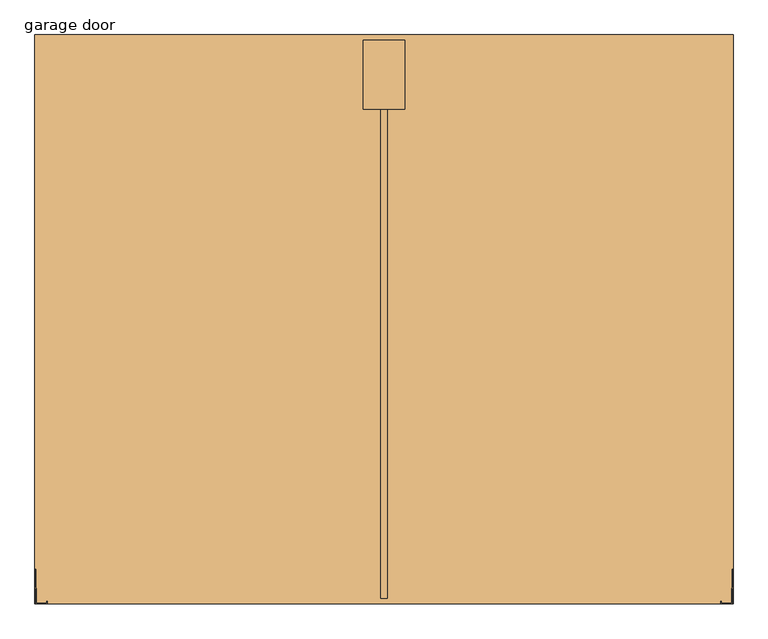
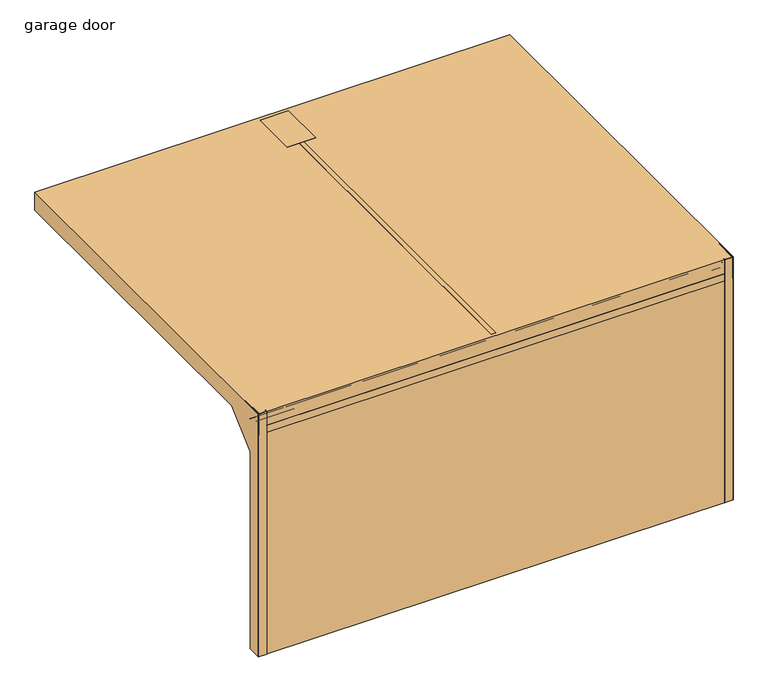
"""IFC4 building model written with IfcOpenShell, lengths in millimetres: door geometry, Sectional_Door_LPU_RU : garage door."""

from ifc_helpers import new_model, si_unit, point, frame, frame_2d, origin, origin_with_axes, place, context, project, spatial, polyline, circle_curve, trimmed, segment, composite_curve, outline, extrude, faceted_brep, source, transform, mapped, element, save
from ifc_brep_helpers import plane_surface, cylinder_surface, revolved_surface, advanced_brep


def garage_door_3c0e62b6(model_context):
    return source(origin(), model_context, "Body", "SolidModel", [
        extrude(outline(polyline([(-1601.2472293, 2039.6377448), (-1628.6278097, 2039.6377448), (-1628.6278097, 2002.03125), (-1637.0303432, 2002.03125), (-1637.0303432, 2490.0), (-1629.0303432, 2490.0), (-1629.0303432, 2512.7083202), (-1605.0303432, 2535.1762842), (-1605.0303432, 2490.0), (-1595.0303432, 2490.0), (-1595.0303432, 2015.0), (-1601.2472293, 2015.0), (-1601.2472293, 2039.6377448)])), frame((-2458.4, 0.0, 0.0), z_axis=(1.0, 0.0, 0.0), x_axis=(0.0, 1.0, 0.0)), (0.0, 0.0, 1.0), 4916.8),
        extrude(outline(polyline([(-1601.2472293, 1539.6377448), (-1628.6278097, 1539.6377448), (-1628.6278097, 1502.03125), (-1637.0303432, 1502.03125), (-1637.0303432, 1990.0), (-1629.0303432, 1990.0), (-1629.0303432, 2012.7083202), (-1605.0303432, 2035.1762842), (-1605.0303432, 1990.0), (-1595.0303432, 1990.0), (-1595.0303432, 1515.0), (-1601.2472293, 1515.0), (-1601.2472293, 1539.6377448)])), frame((-2458.4, 0.0, 0.0), z_axis=(1.0, 0.0, 0.0), x_axis=(0.0, 1.0, 0.0)), (0.0, 0.0, 1.0), 4916.8),
        extrude(outline(polyline([(-1601.2472293, 1039.6377448), (-1628.6278097, 1039.6377448), (-1628.6278097, 1002.03125), (-1637.0303432, 1002.03125), (-1637.0303432, 1490.0), (-1629.0303432, 1490.0), (-1629.0303432, 1512.7083202), (-1605.0303432, 1535.1762842), (-1605.0303432, 1490.0), (-1595.0303432, 1490.0), (-1595.0303432, 1015.0), (-1601.2472293, 1015.0), (-1601.2472293, 1039.6377448)])), frame((-2458.4, 0.0, 0.0), z_axis=(1.0, 0.0, 0.0), x_axis=(0.0, 1.0, 0.0)), (0.0, 0.0, 1.0), 4916.8),
        extrude(outline(polyline([(-1601.2472293, 539.6377448), (-1628.6278097, 539.6377448), (-1628.6278097, 502.03125), (-1637.0303432, 502.03125), (-1637.0303432, 990.0), (-1629.0303432, 990.0), (-1629.0303432, 1012.7083202), (-1605.0303432, 1035.1762842), (-1605.0303432, 990.0), (-1595.0303432, 990.0), (-1595.0303432, 515.0), (-1601.2472293, 515.0), (-1601.2472293, 539.6377448)])), frame((-2458.4, 0.0, 0.0), z_axis=(1.0, 0.0, 0.0), x_axis=(0.0, 1.0, 0.0)), (0.0, 0.0, 1.0), 4916.8),
        extrude(outline(polyline([(-150.0, 2425.9696568), (150.0, 2425.9696568), (150.0, 1925.9696568), (-150.0, 1925.9696568), (-150.0, 2425.9696568)])), frame((0.0, 0.0, 2595.0), z_axis=(0.0, 0.0, 1.0), x_axis=(1.0, 0.0, 0.0)), (0.0, 0.0, 1.0), 140.0),
        extrude(outline(polyline([(2523.4003172, -1659.0303432), (2438.4, -1659.0303432), (2438.4, -1638.7178432), (2441.7654545, -1638.7178432), (2441.7654545, -1655.2208416), (2519.9628172, -1655.2208416), (2519.9628172, -1544.4759666), (2524.739741, -1539.6990428), (2528.2752749, -1543.2345767), (2523.4003172, -1548.1095345), (2523.4003172, -1659.0303432)])), origin_with_axes(), (0.0, 0.0, 1.0), 2735.0),
        extrude(outline(polyline([(-2523.4003172, -1659.0303432), (-2523.4003172, -1548.1095345), (-2528.2752749, -1543.2345767), (-2524.739741, -1539.6990428), (-2519.9628172, -1544.4759666), (-2519.9628172, -1655.2208416), (-2441.7654545, -1655.2208416), (-2441.7654545, -1638.7178432), (-2438.4, -1638.7178432), (-2438.4, -1659.0303432), (-2523.4003172, -1659.0303432)])), origin_with_axes(), (0.0, 0.0, 1.0), 2735.0),
        extrude(outline(polyline([(-1408.7178432, 2735.0), (-1408.7178432, 2595.0), (-1548.1095345, 2494.9608265), (-1659.0303432, 2494.9608265), (-1659.0303432, 2735.0), (-1408.7178432, 2735.0)])), frame((2523.4003172, 0.0, 0.0), z_axis=(1.0, 0.0, 0.0), x_axis=(0.0, 1.0, 0.0)), (0.0, 0.0, 1.0), 3.7125221),
        extrude(outline(polyline([(-1408.7178432, 2735.0), (-1408.7178432, 2595.0), (-1548.1095345, 2494.9608265), (-1659.0303432, 2494.9608265), (-1659.0303432, 2735.0), (-1408.7178432, 2735.0)])), frame((-2527.1128393, 0.0, 0.0), z_axis=(1.0, 0.0, 0.0), x_axis=(0.0, 1.0, 0.0)), (0.0, 0.0, 1.0), 3.7125221),
        extrude(outline(polyline([(2518.4, 1286.6844584), (-2518.4, 1286.6844584), (-2518.4, 1351.6844584), (2518.4, 1351.6844584), (2518.4, 1286.6844584)])), frame((0.0, 0.0, 2687.5), z_axis=(0.0, 0.0, 1.0), x_axis=(1.0, 0.0, 0.0)), (0.0, 0.0, 1.0), 2.5),
        extrude(outline(polyline([(-1659.0303432, 2580.0), (-1638.737141, 2580.0), (-1638.737141, 2565.0), (-1640.5687539, 2565.0), (-1640.5687539, 2577.8988964), (-1657.1312539, 2577.8988964), (-1657.1312539, 2502.7049207), (-1640.5687539, 2502.7049207), (-1640.5687539, 2515.838061), (-1638.737141, 2515.838061), (-1638.737141, 2500.0), (-1659.0303432, 2500.0), (-1659.0303432, 2580.0)])), frame((-2438.4, 0.0, 0.0), z_axis=(1.0, 0.0, 0.0), x_axis=(0.0, 1.0, 0.0)), (0.0, 0.0, 1.0), 4876.8),
        faceted_brep([(-2488.4, -1636.7431471, 2607.219103), (-2518.4, -1636.7431471, 2607.219103), (-2518.4, -1601.2258031, 2552.780897), (-2488.4, -1601.2258031, 2552.780897), (-2488.4, -1607.025551, 2561.6702968), (-2490.8606703, -1607.025551, 2561.6702968), (-2490.8606703, -1602.9273959, 2555.3889654), (-2515.8606703, -1602.9273959, 2555.3889654), (-2515.8606703, -1635.7126366, 2605.6396171), (-2490.8606703, -1635.7126366, 2605.6396171), (-2490.8606703, -1631.2789403, 2598.8439944), (-2488.4, -1631.2789403, 2598.8439944), (-2488.4, 1350.9696568, 2687.5), (-2488.4, 1350.9696568, 2677.5), (-2490.8606703, 1350.9696568, 2677.5), (-2490.8606703, 1350.9696568, 2685.6140711), (-2515.8606703, 1350.9696568, 2685.6140711), (-2515.8606703, 1350.9696568, 2625.6140711), (-2490.8606703, 1350.9696568, 2625.6140711), (-2490.8606703, 1350.9696568, 2633.1140711), (-2488.4, 1350.9696568, 2633.1140711), (-2488.4, 1350.9696568, 2622.5), (-2518.4, 1350.9696568, 2622.5), (-2518.4, 1350.9696568, 2687.5), (-2490.8606703, -1510.7211691, 2677.5), (-2488.4, -1510.7211691, 2677.5), (-2515.8606703, -1513.1340507, 2685.6140711), (-2490.8606703, -1513.1340507, 2685.6140711), (-2490.8606703, -1495.2918483, 2625.6140711), (-2515.8606703, -1495.2918483, 2625.6140711), (-2488.4, -1497.5221236, 2633.1140711), (-2490.8606703, -1497.5221236, 2633.1140711), (-2518.4, -1494.3658169, 2622.5), (-2488.4, -1494.3658169, 2622.5), (-2488.4, -1513.6948695, 2687.5), (-2518.4, -1513.6948695, 2687.5)], [[[0, 1, 2, 3, 4, 5, 6, 7, 8, 9, 10, 11]], [[12, 13, 14, 15, 16, 17, 18, 19, 20, 21, 22, 23]], [[24, 14, 13, 25]], [[26, 16, 15, 27]], [[28, 18, 17, 29]], [[30, 20, 19, 31]], [[32, 22, 21, 33]], [[34, 12, 23, 35]], [[11, 25, 13, 12, 34, 0]], [[10, 24, 25, 11]], [[9, 27, 15, 14, 24, 10]], [[8, 26, 27, 9]], [[7, 29, 17, 16, 26, 8]], [[6, 28, 29, 7]], [[5, 31, 19, 18, 28, 6]], [[4, 30, 31, 5]], [[3, 33, 21, 20, 30, 4]], [[2, 32, 33, 3]], [[1, 35, 23, 22, 32, 2]], [[0, 34, 35, 1]]]),
        faceted_brep([(2488.4, -1636.7431471, 2607.219103), (2488.4, -1631.2789403, 2598.8439944), (2490.8606703, -1631.2789403, 2598.8439944), (2490.8606703, -1635.7126366, 2605.6396171), (2515.8606703, -1635.7126366, 2605.6396171), (2515.8606703, -1602.9273959, 2555.3889654), (2490.8606703, -1602.9273959, 2555.3889654), (2490.8606703, -1607.025551, 2561.6702968), (2488.4, -1607.025551, 2561.6702968), (2488.4, -1601.2258031, 2552.780897), (2518.4, -1601.2258031, 2552.780897), (2518.4, -1636.7431471, 2607.219103), (2488.4, 1350.9696568, 2687.5), (2518.4, 1350.9696568, 2687.5), (2518.4, 1350.9696568, 2622.5), (2488.4, 1350.9696568, 2622.5), (2488.4, 1350.9696568, 2633.1140711), (2490.8606703, 1350.9696568, 2633.1140711), (2490.8606703, 1350.9696568, 2625.6140711), (2515.8606703, 1350.9696568, 2625.6140711), (2515.8606703, 1350.9696568, 2685.6140711), (2490.8606703, 1350.9696568, 2685.6140711), (2490.8606703, 1350.9696568, 2677.5), (2488.4, 1350.9696568, 2677.5), (2518.4, -1513.6948695, 2687.5), (2488.4, -1513.6948695, 2687.5), (2488.4, -1494.3658169, 2622.5), (2518.4, -1494.3658169, 2622.5), (2490.8606703, -1497.5221236, 2633.1140711), (2488.4, -1497.5221236, 2633.1140711), (2515.8606703, -1495.2918483, 2625.6140711), (2490.8606703, -1495.2918483, 2625.6140711), (2490.8606703, -1513.1340507, 2685.6140711), (2515.8606703, -1513.1340507, 2685.6140711), (2488.4, -1510.7211691, 2677.5), (2490.8606703, -1510.7211691, 2677.5)], [[[0, 1, 2, 3, 4, 5, 6, 7, 8, 9, 10, 11]], [[12, 13, 14, 15, 16, 17, 18, 19, 20, 21, 22, 23]], [[24, 13, 12, 25]], [[26, 15, 14, 27]], [[28, 17, 16, 29]], [[30, 19, 18, 31]], [[32, 21, 20, 33]], [[34, 23, 22, 35]], [[11, 24, 25, 0]], [[10, 27, 14, 13, 24, 11]], [[9, 26, 27, 10]], [[8, 29, 16, 15, 26, 9]], [[7, 28, 29, 8]], [[6, 31, 18, 17, 28, 7]], [[5, 30, 31, 6]], [[4, 33, 20, 19, 30, 5]], [[3, 32, 33, 4]], [[2, 35, 22, 21, 32, 3]], [[1, 34, 35, 2]], [[0, 25, 12, 23, 34, 1]]]),
        advanced_brep(
        [(2488.4, -1616.5303432, 0.0), (2488.4, -1606.5303432, 0.0), (2490.8606703, -1606.5303432, 0.0), (2490.8606703, -1614.6444143, 0.0), (2515.8606703, -1614.6444143, 0.0), (2515.8606703, -1554.6444143, 0.0), (2490.8606703, -1554.6444143, 0.0), (2490.8606703, -1562.1444143, 0.0), (2488.4, -1562.1444143, 0.0), (2488.4, -1551.5303432, 0.0), (2518.4, -1551.5303432, 0.0), (2518.4, -1616.5303432, 0.0), (2488.4, -1562.1444143, 2280.0), (2488.4, -1284.0303432, 2558.1140711), (2488.4, 1350.9696568, 2558.1140711), (2488.4, 1350.9696568, 2547.5), (2488.4, -1284.0303432, 2547.5), (2488.4, -1551.5303432, 2280.0), (2490.8606703, -1562.1444143, 2280.0), (2490.8606703, -1284.0303432, 2558.1140711), (2488.4, 1350.9696568, 2612.5), (2518.4, 1350.9696568, 2612.5), (2518.4, 1350.9696568, 2547.5), (2490.8606703, 1350.9696568, 2558.1140711), (2490.8606703, 1350.9696568, 2550.6140711), (2515.8606703, 1350.9696568, 2550.6140711), (2515.8606703, 1350.9696568, 2610.6140711), (2490.8606703, 1350.9696568, 2610.6140711), (2490.8606703, 1350.9696568, 2602.5), (2488.4, 1350.9696568, 2602.5), (2488.4, -1616.5303432, 2280.0), (2488.4, -1284.0303432, 2612.5), (2488.4, -1284.0303432, 2602.5), (2488.4, -1606.5303432, 2280.0), (2490.8606703, -1606.5303432, 2280.0), (2490.8606703, -1284.0303432, 2602.5), (2490.8606703, -1284.0303432, 2610.6140711), (2490.8606703, -1614.6444143, 2280.0), (2515.8606703, -1614.6444143, 2280.0), (2515.8606703, -1284.0303432, 2610.6140711), (2515.8606703, -1284.0303432, 2550.6140711), (2515.8606703, -1554.6444143, 2280.0), (2490.8606703, -1554.6444143, 2280.0), (2490.8606703, -1284.0303432, 2550.6140711), (2518.4, -1551.5303432, 2280.0), (2518.4, -1284.0303432, 2547.5), (2518.4, -1284.0303432, 2612.5), (2518.4, -1616.5303432, 2280.0)],
        [
            (0, 1),
            (1, 2),
            (2, 3),
            (3, 4),
            (4, 5),
            (5, 6),
            (6, 7),
            (7, 8),
            (8, 9),
            (9, 10),
            (10, 11),
            (11, 0),
            (8, 12),
            (12, 13, circle_curve(frame((2488.4, -1284.0303432, 2280.0), z_axis=(-1.0, 0.0, 0.0), x_axis=(0.0, -1.0, 0.0)), 278.1140711)),
            (13, 14),
            (14, 15),
            (15, 16),
            (16, 17, circle_curve(frame((2488.4, -1284.0303432, 2280.0), z_axis=(1.0, 0.0, 0.0), x_axis=(0.0, -1.0, 0.0)), 267.5)),
            (17, 9),
            (7, 18),
            (18, 12),
            (19, 13),
            (18, 19, circle_curve(frame((2490.8606703, -1284.0303432, 2280.0), z_axis=(-1.0, 0.0, 0.0), x_axis=(0.0, -1.0, 0.0)), 278.1140711)),
            (20, 21),
            (21, 22),
            (22, 15),
            (14, 23),
            (23, 24),
            (24, 25),
            (25, 26),
            (26, 27),
            (27, 28),
            (28, 29),
            (29, 20),
            (19, 23),
            (0, 30),
            (30, 31, circle_curve(frame((2488.4, -1284.0303432, 2280.0), z_axis=(-1.0, 0.0, 0.0), x_axis=(0.0, -1.0, 0.0)), 332.5)),
            (31, 20),
            (29, 32),
            (32, 33, circle_curve(frame((2488.4, -1284.0303432, 2280.0), z_axis=(1.0, 0.0, 0.0), x_axis=(0.0, -1.0, 0.0)), 322.5)),
            (33, 1),
            (33, 34),
            (34, 2),
            (34, 35, circle_curve(frame((2490.8606703, -1284.0303432, 2280.0), z_axis=(-1.0, 0.0, 0.0), x_axis=(0.0, -1.0, 0.0)), 322.5)),
            (35, 28),
            (27, 36),
            (36, 37, circle_curve(frame((2490.8606703, -1284.0303432, 2280.0), z_axis=(1.0, 0.0, 0.0), x_axis=(0.0, -1.0, 0.0)), 330.6140711)),
            (37, 3),
            (37, 38),
            (38, 4),
            (38, 39, circle_curve(frame((2515.8606703, -1284.0303432, 2280.0), z_axis=(-1.0, 0.0, 0.0), x_axis=(0.0, -1.0, 0.0)), 330.6140711)),
            (39, 26),
            (25, 40),
            (40, 41, circle_curve(frame((2515.8606703, -1284.0303432, 2280.0), z_axis=(1.0, 0.0, 0.0), x_axis=(0.0, -1.0, 0.0)), 270.6140711)),
            (41, 5),
            (41, 42),
            (42, 6),
            (42, 43, circle_curve(frame((2490.8606703, -1284.0303432, 2280.0), z_axis=(-1.0, 0.0, 0.0), x_axis=(0.0, -1.0, 0.0)), 270.6140711)),
            (43, 24),
            (17, 44),
            (44, 10),
            (44, 45, circle_curve(frame((2518.4, -1284.0303432, 2280.0), z_axis=(-1.0, 0.0, 0.0), x_axis=(0.0, -1.0, 0.0)), 267.5)),
            (45, 22),
            (21, 46),
            (46, 47, circle_curve(frame((2518.4, -1284.0303432, 2280.0), z_axis=(1.0, 0.0, 0.0), x_axis=(0.0, -1.0, 0.0)), 332.5)),
            (47, 11),
            (47, 30),
            (32, 35),
            (36, 39),
            (40, 43),
            (16, 45),
            (46, 31),
        ],
        [
            plane_surface(frame((2438.4, -1584.0303432, 0.0), z_axis=(0.0, 0.0, -1.0), x_axis=(1.0, 0.0, 0.0))),
            plane_surface(frame((2488.4, -1551.5303432, 0.0), z_axis=(-1.0, 0.0, 0.0), x_axis=(0.0, 0.0, 1.0))),
            plane_surface(frame((2488.4, -1562.1444143, 0.0), z_axis=(0.0, -1.0, 0.0), x_axis=(0.0, 0.0, 1.0))),
            cylinder_surface(frame((2438.4, -1284.0303432, 2280.0), z_axis=(1.0, 0.0, 0.0), x_axis=(0.0, -1.0, 0.0)), 278.1140711),
            plane_surface(frame((2438.4, 1350.9696568, 2580.0), z_axis=(0.0, 1.0, 0.0), x_axis=(1.0, 0.0, 0.0))),
            plane_surface(frame((2488.4, -1284.0303432, 2558.1140711), z_axis=(0.0, 0.0, 1.0), x_axis=(0.0, 1.0, 0.0))),
            plane_surface(frame((2488.4, -1606.5303432, 0.0), z_axis=(-1.0, 0.0, 0.0), x_axis=(0.0, 0.0, 1.0))),
            plane_surface(frame((2490.8606703, -1606.5303432, 0.0), z_axis=(0.0, 1.0, 0.0), x_axis=(0.0, 0.0, 1.0))),
            plane_surface(frame((2490.8606703, -1614.6444143, 0.0), z_axis=(1.0, 0.0, 0.0), x_axis=(0.0, 0.0, 1.0))),
            plane_surface(frame((2515.8606703, -1614.6444143, 0.0), z_axis=(0.0, 1.0, 0.0), x_axis=(0.0, 0.0, 1.0))),
            plane_surface(frame((2515.8606703, -1554.6444143, 0.0), z_axis=(-1.0, 0.0, 0.0), x_axis=(0.0, 0.0, 1.0))),
            plane_surface(frame((2490.8606703, -1554.6444143, 0.0), z_axis=(0.0, -1.0, 0.0), x_axis=(0.0, 0.0, 1.0))),
            plane_surface(frame((2490.8606703, -1562.1444143, 0.0), z_axis=(1.0, 0.0, 0.0), x_axis=(0.0, 0.0, 1.0))),
            plane_surface(frame((2518.4, -1551.5303432, 0.0), z_axis=(0.0, 1.0, 0.0), x_axis=(0.0, 0.0, 1.0))),
            plane_surface(frame((2518.4, -1616.5303432, 0.0), z_axis=(1.0, 0.0, 0.0), x_axis=(0.0, 0.0, 1.0))),
            plane_surface(frame((2488.4, -1616.5303432, 0.0), z_axis=(0.0, -1.0, 0.0), x_axis=(0.0, 0.0, 1.0))),
            revolved_surface(polyline([(2490.8606703, -1606.5303432, 2280.0), (2488.4, -1606.5303432, 2280.0)]), (2438.4, -1284.0303432, 2280.0), (1.0, 0.0, 0.0)),
            revolved_surface(polyline([(2515.8606703, -1614.6444143, 2280.0), (2490.8606703, -1614.6444143, 2280.0)]), (2438.4, -1284.0303432, 2280.0), (1.0, 0.0, 0.0)),
            cylinder_surface(frame((2438.4, -1284.0303432, 2280.0), z_axis=(1.0, 0.0, 0.0), x_axis=(0.0, -1.0, 0.0)), 270.6140711),
            revolved_surface(polyline([(2518.4, -1551.5303432, 2280.0), (2488.4, -1551.5303432, 2280.0)]), (2438.4, -1284.0303432, 2280.0), (1.0, 0.0, 0.0)),
            cylinder_surface(frame((2438.4, -1284.0303432, 2280.0), z_axis=(1.0, 0.0, 0.0), x_axis=(0.0, -1.0, 0.0)), 332.5),
            plane_surface(frame((2490.8606703, -1284.0303432, 2602.5), z_axis=(0.0, 0.0, -1.0), x_axis=(0.0, 1.0, 0.0))),
            plane_surface(frame((2515.8606703, -1284.0303432, 2610.6140711), z_axis=(0.0, 0.0, -1.0), x_axis=(0.0, 1.0, 0.0))),
            plane_surface(frame((2490.8606703, -1284.0303432, 2550.6140711), z_axis=(0.0, 0.0, 1.0), x_axis=(0.0, 1.0, 0.0))),
            plane_surface(frame((2518.4, -1284.0303432, 2547.5), z_axis=(0.0, 0.0, -1.0), x_axis=(0.0, 1.0, 0.0))),
            plane_surface(frame((2488.4, -1284.0303432, 2612.5), z_axis=(0.0, 0.0, 1.0), x_axis=(0.0, 1.0, 0.0))),
        ],
        [
            (0, [[1, 2, 3, 4, 5, 6, 7, 8, 9, 10, 11, 12]]),
            (1, [[13, 14, 15, 16, 17, 18, 19, -9]]),
            (2, [[20, 21, -13, -8]]),
            (3, [[22, -14, -21, 23]]),
            (4, [[24, 25, 26, -16, 27, 28, 29, 30, 31, 32, 33, 34]]),
            (5, [[35, -27, -15, -22]]),
            (6, [[36, 37, 38, -34, 39, 40, 41, -1]]),
            (7, [[-41, 42, 43, -2]]),
            (8, [[-43, 44, 45, -32, 46, 47, 48, -3]]),
            (9, [[-48, 49, 50, -4]]),
            (10, [[-50, 51, 52, -30, 53, 54, 55, -5]]),
            (11, [[-55, 56, 57, -6]]),
            (12, [[-57, 58, 59, -28, -35, -23, -20, -7]]),
            (13, [[-19, 60, 61, -10]]),
            (14, [[-61, 62, 63, -25, 64, 65, 66, -11]]),
            (15, [[-66, 67, -36, -12]]),
            (16, [[68, -44, -42, -40]]),
            (17, [[69, -51, -49, -47]]),
            (18, [[70, -58, -56, -54]]),
            (19, [[71, -62, -60, -18]]),
            (20, [[72, -37, -67, -65]]),
            (21, [[-39, -33, -45, -68]]),
            (22, [[-46, -31, -52, -69]]),
            (23, [[-53, -29, -59, -70]]),
            (24, [[-17, -26, -63, -71]]),
            (25, [[-64, -24, -38, -72]]),
        ],
    ),
        advanced_brep(
        [(-2488.4, -1616.5303432, 0.0), (-2518.4, -1616.5303432, 0.0), (-2518.4, -1551.5303432, 0.0), (-2488.4, -1551.5303432, 0.0), (-2488.4, -1562.1444143, 0.0), (-2490.8606703, -1562.1444143, 0.0), (-2490.8606703, -1554.6444143, 0.0), (-2515.8606703, -1554.6444143, 0.0), (-2515.8606703, -1614.6444143, 0.0), (-2490.8606703, -1614.6444143, 0.0), (-2490.8606703, -1606.5303432, 0.0), (-2488.4, -1606.5303432, 0.0), (-2518.4, -1616.5303432, 2280.0), (-2518.4, -1284.0303432, 2612.5), (-2518.4, 1350.9696568, 2612.5), (-2518.4, 1350.9696568, 2547.5), (-2518.4, -1284.0303432, 2547.5), (-2518.4, -1551.5303432, 2280.0), (-2488.4, -1551.5303432, 2280.0), (-2488.4, -1606.5303432, 2280.0), (-2488.4, -1284.0303432, 2602.5), (-2488.4, 1350.9696568, 2602.5), (-2488.4, 1350.9696568, 2612.5), (-2488.4, -1284.0303432, 2612.5), (-2488.4, -1616.5303432, 2280.0), (-2490.8606703, -1606.5303432, 2280.0), (-2490.8606703, -1614.6444143, 2280.0), (-2490.8606703, -1284.0303432, 2610.6140711), (-2490.8606703, 1350.9696568, 2610.6140711), (-2490.8606703, 1350.9696568, 2602.5), (-2490.8606703, -1284.0303432, 2602.5), (-2515.8606703, -1614.6444143, 2280.0), (-2515.8606703, -1554.6444143, 2280.0), (-2515.8606703, -1284.0303432, 2550.6140711), (-2515.8606703, 1350.9696568, 2550.6140711), (-2515.8606703, 1350.9696568, 2610.6140711), (-2515.8606703, -1284.0303432, 2610.6140711), (-2490.8606703, -1554.6444143, 2280.0), (-2490.8606703, -1562.1444143, 2280.0), (-2490.8606703, -1284.0303432, 2558.1140711), (-2490.8606703, 1350.9696568, 2558.1140711), (-2490.8606703, 1350.9696568, 2550.6140711), (-2490.8606703, -1284.0303432, 2550.6140711), (-2488.4, 1350.9696568, 2558.1140711), (-2488.4, 1350.9696568, 2547.5), (-2488.4, -1284.0303432, 2547.5), (-2488.4, -1562.1444143, 2280.0), (-2488.4, -1284.0303432, 2558.1140711)],
        [
            (0, 1),
            (1, 2),
            (2, 3),
            (3, 4),
            (4, 5),
            (5, 6),
            (6, 7),
            (7, 8),
            (8, 9),
            (9, 10),
            (10, 11),
            (11, 0),
            (1, 12),
            (12, 13, circle_curve(frame((-2518.4, -1284.0303432, 2280.0), z_axis=(-1.0, 0.0, 0.0), x_axis=(0.0, -1.0, 0.0)), 332.5)),
            (13, 14),
            (14, 15),
            (15, 16),
            (16, 17, circle_curve(frame((-2518.4, -1284.0303432, 2280.0), z_axis=(1.0, 0.0, 0.0), x_axis=(0.0, -1.0, 0.0)), 267.5)),
            (17, 2),
            (17, 18),
            (18, 3),
            (11, 19),
            (19, 20, circle_curve(frame((-2488.4, -1284.0303432, 2280.0), z_axis=(-1.0, 0.0, 0.0), x_axis=(0.0, -1.0, 0.0)), 322.5)),
            (20, 21),
            (21, 22),
            (22, 23),
            (23, 24, circle_curve(frame((-2488.4, -1284.0303432, 2280.0), z_axis=(1.0, 0.0, 0.0), x_axis=(0.0, -1.0, 0.0)), 332.5)),
            (24, 0),
            (10, 25),
            (25, 19),
            (9, 26),
            (26, 27, circle_curve(frame((-2490.8606703, -1284.0303432, 2280.0), z_axis=(-1.0, 0.0, 0.0), x_axis=(0.0, -1.0, 0.0)), 330.6140711)),
            (27, 28),
            (28, 29),
            (29, 30),
            (30, 25, circle_curve(frame((-2490.8606703, -1284.0303432, 2280.0), z_axis=(1.0, 0.0, 0.0), x_axis=(0.0, -1.0, 0.0)), 322.5)),
            (8, 31),
            (31, 26),
            (7, 32),
            (32, 33, circle_curve(frame((-2515.8606703, -1284.0303432, 2280.0), z_axis=(-1.0, 0.0, 0.0), x_axis=(0.0, -1.0, 0.0)), 270.6140711)),
            (33, 34),
            (34, 35),
            (35, 36),
            (36, 31, circle_curve(frame((-2515.8606703, -1284.0303432, 2280.0), z_axis=(1.0, 0.0, 0.0), x_axis=(0.0, -1.0, 0.0)), 330.6140711)),
            (6, 37),
            (37, 32),
            (5, 38),
            (38, 39, circle_curve(frame((-2490.8606703, -1284.0303432, 2280.0), z_axis=(-1.0, 0.0, 0.0), x_axis=(0.0, -1.0, 0.0)), 278.1140711)),
            (39, 40),
            (40, 41),
            (41, 42),
            (42, 37, circle_curve(frame((-2490.8606703, -1284.0303432, 2280.0), z_axis=(1.0, 0.0, 0.0), x_axis=(0.0, -1.0, 0.0)), 270.6140711)),
            (24, 12),
            (21, 29),
            (28, 35),
            (34, 41),
            (40, 43),
            (43, 44),
            (44, 15),
            (14, 22),
            (44, 45),
            (45, 16),
            (20, 30),
            (27, 36),
            (33, 42),
            (13, 23),
            (45, 18, circle_curve(frame((-2488.4, -1284.0303432, 2280.0), z_axis=(1.0, 0.0, 0.0), x_axis=(0.0, -1.0, 0.0)), 267.5)),
            (4, 46),
            (46, 38),
            (43, 47),
            (47, 46, circle_curve(frame((-2488.4, -1284.0303432, 2280.0), z_axis=(1.0, 0.0, 0.0), x_axis=(0.0, -1.0, 0.0)), 278.1140711)),
            (47, 39),
        ],
        [
            plane_surface(frame((-2438.4, -1584.0303432, 0.0), z_axis=(0.0, 0.0, -1.0), x_axis=(1.0, 0.0, 0.0))),
            plane_surface(frame((-2518.4, -1551.5303432, 0.0), z_axis=(-1.0, 0.0, 0.0), x_axis=(0.0, 0.0, 1.0))),
            plane_surface(frame((-2488.4, -1551.5303432, 0.0), z_axis=(0.0, 1.0, 0.0), x_axis=(0.0, 0.0, 1.0))),
            plane_surface(frame((-2488.4, -1616.5303432, 0.0), z_axis=(1.0, 0.0, 0.0), x_axis=(0.0, 0.0, 1.0))),
            plane_surface(frame((-2488.4, -1606.5303432, 0.0), z_axis=(0.0, 1.0, 0.0), x_axis=(0.0, 0.0, 1.0))),
            plane_surface(frame((-2490.8606703, -1606.5303432, 0.0), z_axis=(-1.0, 0.0, 0.0), x_axis=(0.0, 0.0, 1.0))),
            plane_surface(frame((-2490.8606703, -1614.6444143, 0.0), z_axis=(0.0, 1.0, 0.0), x_axis=(0.0, 0.0, 1.0))),
            plane_surface(frame((-2515.8606703, -1614.6444143, 0.0), z_axis=(1.0, 0.0, 0.0), x_axis=(0.0, 0.0, 1.0))),
            plane_surface(frame((-2515.8606703, -1554.6444143, 0.0), z_axis=(0.0, -1.0, 0.0), x_axis=(0.0, 0.0, 1.0))),
            plane_surface(frame((-2490.8606703, -1554.6444143, 0.0), z_axis=(-1.0, 0.0, 0.0), x_axis=(0.0, 0.0, 1.0))),
            plane_surface(frame((-2518.4, -1616.5303432, 0.0), z_axis=(0.0, -1.0, 0.0), x_axis=(0.0, 0.0, 1.0))),
            plane_surface(frame((-2438.4, 1350.9696568, 2580.0), z_axis=(0.0, 1.0, 0.0), x_axis=(1.0, 0.0, 0.0))),
            plane_surface(frame((-2488.4, -1284.0303432, 2547.5), z_axis=(0.0, 0.0, -1.0), x_axis=(0.0, 1.0, 0.0))),
            plane_surface(frame((-2488.4, -1284.0303432, 2602.5), z_axis=(0.0, 0.0, -1.0), x_axis=(0.0, 1.0, 0.0))),
            plane_surface(frame((-2490.8606703, -1284.0303432, 2610.6140711), z_axis=(0.0, 0.0, -1.0), x_axis=(0.0, 1.0, 0.0))),
            plane_surface(frame((-2515.8606703, -1284.0303432, 2550.6140711), z_axis=(0.0, 0.0, 1.0), x_axis=(0.0, 1.0, 0.0))),
            plane_surface(frame((-2518.4, -1284.0303432, 2612.5), z_axis=(0.0, 0.0, 1.0), x_axis=(0.0, 1.0, 0.0))),
            revolved_surface(polyline([(-2488.4, -1551.5303432, 2280.0), (-2518.4, -1551.5303432, 2280.0)]), (-2438.4, -1284.0303432, 2280.0), (1.0, 0.0, 0.0)),
            revolved_surface(polyline([(-2488.4, -1606.5303432, 2280.0), (-2490.8606703, -1606.5303432, 2280.0)]), (-2438.4, -1284.0303432, 2280.0), (1.0, 0.0, 0.0)),
            revolved_surface(polyline([(-2490.8606703, -1614.6444143, 2280.0), (-2515.8606703, -1614.6444143, 2280.0)]), (-2438.4, -1284.0303432, 2280.0), (1.0, 0.0, 0.0)),
            cylinder_surface(frame((-2438.4, -1284.0303432, 2280.0), z_axis=(1.0, 0.0, 0.0), x_axis=(0.0, -1.0, 0.0)), 270.6140711),
            cylinder_surface(frame((-2438.4, -1284.0303432, 2280.0), z_axis=(1.0, 0.0, 0.0), x_axis=(0.0, -1.0, 0.0)), 332.5),
            plane_surface(frame((-2490.8606703, -1562.1444143, 0.0), z_axis=(0.0, -1.0, 0.0), x_axis=(0.0, 0.0, 1.0))),
            plane_surface(frame((-2488.4, -1562.1444143, 0.0), z_axis=(1.0, 0.0, 0.0), x_axis=(0.0, 0.0, 1.0))),
            cylinder_surface(frame((-2438.4, -1284.0303432, 2280.0), z_axis=(1.0, 0.0, 0.0), x_axis=(0.0, -1.0, 0.0)), 278.1140711),
            plane_surface(frame((-2490.8606703, -1284.0303432, 2558.1140711), z_axis=(0.0, 0.0, 1.0), x_axis=(0.0, 1.0, 0.0))),
        ],
        [
            (0, [[1, 2, 3, 4, 5, 6, 7, 8, 9, 10, 11, 12]]),
            (1, [[13, 14, 15, 16, 17, 18, 19, -2]]),
            (2, [[-19, 20, 21, -3]]),
            (3, [[22, 23, 24, 25, 26, 27, 28, -12]]),
            (4, [[29, 30, -22, -11]]),
            (5, [[31, 32, 33, 34, 35, 36, -29, -10]]),
            (6, [[37, 38, -31, -9]]),
            (7, [[39, 40, 41, 42, 43, 44, -37, -8]]),
            (8, [[45, 46, -39, -7]]),
            (9, [[47, 48, 49, 50, 51, 52, -45, -6]]),
            (10, [[-28, 53, -13, -1]]),
            (11, [[-25, 54, -34, 55, -42, 56, -50, 57, 58, 59, -16, 60]]),
            (12, [[-17, -59, 61, 62]]),
            (13, [[-35, -54, -24, 63]]),
            (14, [[-43, -55, -33, 64]]),
            (15, [[-51, -56, -41, 65]]),
            (16, [[-26, -60, -15, 66]]),
            (17, [[-62, 67, -20, -18]]),
            (18, [[-63, -23, -30, -36]]),
            (19, [[-64, -32, -38, -44]]),
            (20, [[-65, -40, -46, -52]]),
            (21, [[-66, -14, -53, -27]]),
            (22, [[68, 69, -47, -5]]),
            (23, [[-21, -67, -61, -58, 70, 71, -68, -4]]),
            (24, [[72, -48, -69, -71]]),
            (25, [[-70, -57, -49, -72]]),
        ],
    ),
        extrude(outline(polyline([(25.0, -1618.9844751), (-25.0, -1618.9844751), (-25.0, 1925.9696568), (25.0, 1925.9696568), (25.0, -1618.9844751)])), frame((0.0, 0.0, 2705.0), z_axis=(0.0, 0.0, 1.0), x_axis=(1.0, 0.0, 0.0)), (0.0, 0.0, 1.0), 30.0),
        extrude(outline(composite_curve([segment(trimmed(circle_curve(frame_2d((-1479.0303432, 2580.0)), 10.0), [point((-1469.0303432, 2580.0))], [point((-1489.0303432, 2580.0))], False, "CARTESIAN"), True, "CONTINUOUS"), segment(trimmed(circle_curve(frame_2d((-1479.0303432, 2580.0)), 10.0), [point((-1489.0303432, 2580.0))], [point((-1469.0303432, 2580.0))], False, "CARTESIAN"), True, "CONTINUOUS")], self_intersect=False)), frame((-2518.4, 0.0, 0.0), z_axis=(1.0, 0.0, 0.0), x_axis=(0.0, 1.0, 0.0)), (0.0, 0.0, 1.0), 5036.8),
        extrude(outline(composite_curve([segment(trimmed(circle_curve(frame_2d((-1479.0303432, 2580.0)), 50.0), [point((-1429.0303432, 2580.0))], [point((-1529.0303432, 2580.0))], False, "CARTESIAN"), True, "CONTINUOUS"), segment(trimmed(circle_curve(frame_2d((-1479.0303432, 2580.0)), 50.0), [point((-1529.0303432, 2580.0))], [point((-1429.0303432, 2580.0))], False, "CARTESIAN"), True, "CONTINUOUS")], self_intersect=False)), frame((-2468.4, 0.0, 0.0), z_axis=(1.0, 0.0, 0.0), x_axis=(0.0, 1.0, 0.0)), (0.0, 0.0, 1.0), 400.0),
        extrude(outline(composite_curve([segment(trimmed(circle_curve(frame_2d((-1479.0303432, 2580.0)), 50.0), [point((-1429.0303432, 2580.0))], [point((-1529.0303432, 2580.0))], False, "CARTESIAN"), True, "CONTINUOUS"), segment(trimmed(circle_curve(frame_2d((-1479.0303432, 2580.0)), 50.0), [point((-1529.0303432, 2580.0))], [point((-1429.0303432, 2580.0))], False, "CARTESIAN"), True, "CONTINUOUS")], self_intersect=False)), frame((2068.4, 0.0, 0.0), z_axis=(1.0, 0.0, 0.0), x_axis=(0.0, 1.0, 0.0)), (0.0, 0.0, 1.0), 400.0),
        extrude(outline(polyline([(-1659.0303432, 2735.0), (2465.9696568, 2735.0), (2465.9696568, 2530.0), (-1169.0303432, 2530.0), (-1504.0303432, 2215.0), (-1504.0303432, 0.0), (-1659.0303432, 0.0), (-1659.0303432, 2735.0)])), frame((-2528.4, 0.0, 0.0), z_axis=(1.0, 0.0, 0.0), x_axis=(0.0, 1.0, 0.0)), (0.0, 0.0, 1.0), 5056.8),
        extrude(outline(polyline([(-1601.2472293, 39.6377448), (-1628.6278097, 39.6377448), (-1628.6278097, 2.03125), (-1637.0303432, 2.03125), (-1637.0303432, 490.0), (-1629.0303432, 490.0), (-1629.0303432, 512.7083202), (-1605.0303432, 535.1762842), (-1605.0303432, 490.0), (-1595.0303432, 490.0), (-1595.0303432, 15.0), (-1601.2472293, 15.0), (-1601.2472293, 39.6377448)])), frame((-2458.4, 0.0, 0.0), z_axis=(1.0, 0.0, 0.0), x_axis=(0.0, 1.0, 0.0)), (0.0, 0.0, 1.0), 4916.8),
    ])


if __name__ == "__main__":
    model = new_model("IFC4")
    model_context = context("Model", 3, world=origin())
    ifc_project = project(units=[si_unit("LENGTHUNIT", "METRE", prefix="MILLI")], contexts=[model_context])
    site = spatial("IfcSite", under=ifc_project)
    building = spatial("IfcBuilding", under=site)
    placement = place(None, origin())
    garage_door_shape = garage_door_3c0e62b6(model_context)
    element("IfcDoor", 1, ObjectType="Sectional_Door_LPU_RU : garage door", at=placement, inside=building, context=model_context, shape_type="MappedRepresentation", body=[
        mapped(garage_door_shape, transform((0.0, 0.0, 0.0), x_axis=(1.0, 0.0, 0.0), y_axis=(0.0, 1.0, 0.0), z_axis=(0.0, 0.0, 1.0))),
    ])
    save(model, "model.ifc")

# Revit data of these elements
# Type "Sectional_Door_LPU_RU : garage door"
#   Type Mark = "30"
#   hoermann_family_version = "202111"
#   bimsys_family_version = "202111261846"
#   Wärmeschutz = "1.4 W/(m²·K)"
#   Windlastklasse nach EN 12424 = "Класс 3 – (0,7 кН/м2 или 120 км/ч)"
#   Verglasung Typ = "Без остекления"
#   URL 3 = "https://www.hoermann.de/mediacenter/"
#   URL 2 = "https://architektenprogramm.hoermann.de/HAP/entry.php"
#   URL = "https://www.hoermann.de/"
#   Steuerung Typ = "с помощью ручных передатчиков"
#   Schlupftür Typ = "Без порога"
#   Schlupftür Schloss Typ = "Стандартный замок"
#   Schlupftür Panikfunktion Typ = "Отсутствует"
#   Schlupftür Obentürschließer Typ = "Производно – доводчик с шиной скольжения"
#   Schlupftür DIN Richtung Typ = "DIN правый"
#   Schlupftür Bänder Typ = "Скрытые петли"
#   Schlupftür Beschlag innen Typ = "Производно (нажимная ручка U-образной формы)"
#   Schlupftür Beschlag außen Typ = "Без нажимной ручки"
#   Schlupftür Beschlag Material Typ = "Пластмасса черного цвета"
#   Schlupftür Aufschlagsrichtung = "глядя наружу"
#   Schallschutz = "Отсутствует"
#   STLB Leistungsbereich = "Двери / Ворота - Металл"
#   STLB Gewerk = "31"
#   Model = "LPU 42, Секция «Гараж»"
#   Lamellen Tor innen Typ = "С оттиском Stucco"
#   Lamellen Tor außen Typ = "Вудгрейн"
#   Lamellen Profil Typ = "L-гофр"
#   Gewichtsausgleich = "Технология натяжения пружины"
#   Fire Rating = "Отсутствует"
#   Einbruchschutz = "Отсутствует"
#   Einbauort = "Наружные стены"
#   DIN 276 Kostengruppe = "334"
#   CAL_Antrieb = "SupraMatic"
#   Manufacturer = "HÖRMANN"
#   Beschlag Tor Typ = "N-направляющая"
#   Beschichtung Lamellen innen Typ = "RAL 9002"
#   Beschichtung Lamellen außen Typ = "RAL 9016"
#   Antrieb Typ = "Отсутствует"
#   Analytic Construction = "<Keine Auswahl>"
#   Versatz Beschlag Schlupftür = 0' - 3.14961"
#   Torblatt Stärke (Bautiefe) = 0' - 1.65354"
#   Sturzhöhe [instance default] = 0' - 8.26772"
#   Schlupftür Stärke (Bautiefe) = 0' - 1.65354"
#   Schlupftür Lichte Durchgangshöhe [instance default] = 6' - 4.9685"
#   Schlupftür Lichte Durchgangsbreite = 2' - 8.67717"
#   Schlupftür Höhe [instance default] = 6' - 4.9685"
#   Schlupftür Breite = 3' - 1.00787"
#   Schlupftür Bedienelement Höhe = 3' - 5.33858"
#   Platzbedarf Lagerseite = 0' - 0"
#   Platzbedarf Antriebsseite = 0' - 0"
#   Fußbodenaufbau = 0' - 0"
#   Deckenhöhe min. [instance default] = 8' - 10.69291"
#   CAL_MinHöhe = 6' - 1.8189"
#   CAL_MinBreite = 6' - 6.74016"
#   Blende oben Ansichtshöhe = 0' - 0"
#   Rough Height = 8' - 2.4252"
#   Rough Width = 16' - 0"
#   CAL_RasterBreite [instance default] = 1' - 10.8189"
#   CAL_Beschlagsart extra länge = 1' - 8.07874"
#   CAL_Beschlag Extra Abstand = 2' - 5.52756"
#   CAL_PanelPosTop [instance default] = 4' - 11.05512"
#   CAL_Schlupftüre Position - Real [instance default] = 6' - 8.69291"
#   CAL_Schlupftüre Position - Kalkuliert [instance default] = 6' - 8.69291"
#   CAL_Beschlag Schlupftüre Position [instance default] = 2' - 8.71654"
#   CAL_Versatz Schlupftüre [instance default] = 4' - 6.67717"
#   CAL_PanelH_Min = 1' - 1.77953"
#   CAL_PanelH_Max = 3' - 7.30709"
#   CAL_Lamellen seitliche Überlappung = 0' - 0.7874"
#   CAL_Panel Tiefe = 0' - 1.65354"
#   CAL_Panel max. Breite [instance default] = 2' - 6.69291"
#   CAL_Panel Breite [instance default] = 16' - 1.5748"
#   CAL_Lamellen Höhe [instance default] = 1' - 7.68504"
#   CAL_Paneel Wandabstand = 0' - 0.86614"
#   CAL_Antrieb Abstand von Öffnungkopf [instance default] = 0' - 8.46457"
#   CAL_Antrieb Beschlag Breite = 0' - 1.1811"
#   CAL_Antrieb Beschlag Tiefe = 0' - 2.75591"
#   CAL_MaxGrößeSchlupftüre = 13' - 1.48031"
#   CAL_MaxBreite = 19' - 8.22047"
#   CAL_MaxHöhe = 9' - 10.11024"
#   CAL_GlasPanVerPos [instance default] = 3' - 3.37008"
#   Height = 8' - 2.4252"
#   CAL_Extra Horizontal Abstand = 3' - 3.37008"
#   Width = 16' - 0"
#   Verglasung ab Lamelle = 3
#   Verglasung Anzahl verglaster Lamellen = 1
#   Torglieder Anzahl = 5
#   ThermoFrame = no
#   Schlupftüranordnung = 2
#   Замок калитки, тип Id = 1
#   Калитка, функция «антипаника», тип Id = 1
#   Калитка, верхний доводчик, тип Id = 1
#   Калитка, направление открывания по DIN, тип Id = 1
#   Калитка, фурнитура, материал, тип Id = 1
#   Schlupftür = no
#   Minimalen Platzbedarf anzeigen [instance default] = yes
#   CE-Kennzeichen vorhanden = yes
#   Направляющая, ворота, тип Id = 3
#   CAL_TopPanelArray [instance default] = no
#   CAL_Größenwarnung [instance default] = no
#   CAL_FensterPanelAn [instance default] = no
#   CAL_OberPanelSingleAn [instance default] = no
#   CAL_OberPanelReiheAn [instance default] = no
#   CAL_Fehlermeldung anzeigen [instance default] = yes
#   Калитка, фурнитура внутри, тип Id = 1
#   CAL_Schlupftüre für Größe = yes
#   CAL_Fehler Schlupftüre [instance default] = no
#   CAL_Schlupftüre  - Real = no
#   CAL_PanelRasterNumTypeS [instance default] = 8
#   CAL_PanelRasterNumTypeM [instance default] = 6
#   CAL_PanelRasterNumTypeL [instance default] = 4
#   CAL_PanelRasterNumTypeD [instance default] = 5
#   CAL_PanelRasterNum [instance default] = 8
#   CAL_PanelNumberTop - Real [instance default] = 2
#   CAL_PanelNumberBottom - Real [instance default] = 5
#   CAL_Schlupftüre Links [instance default] = no
#   CAL_PanelNumber - Real [instance default] = 5
#   Секции, профиль, тип Id = 1
#   Калитка, фурнитура снаружи, тип Id = 1
#   CAL_Antrieb Id = 1
#   Остекление, тип Id = 0
#   CAL_Fehlermeldung sichtbar [instance default] = no
#   CAL_Schlupftüre für Typ = yes
#   CAL_UnterPanelEinzel = no
#   CAL_UnterPanelReihe = yes
#   Покрытие секций изнутри, тип Id = 1
#   Покрытие секций снаружи, тип Id = 1
#   Тип привода Id = 1
#   Zarge Material = Hörmann - RAL 9002
#   Schlupftür Beschlag Oberfläche = Hörmann - RAL 7004
#   Lamellen Material = Wall Texture, Stucco
#   CAL_Glaspanel Typ LPU [instance default] = element 711548
#   CAL_Glaspanel Typ Familie [instance default] = element 711548
#   CAL_Glaspanel Typ Alu-Rahmen [instance default] = element 711550
#   Остекление, материал = Hörmann - Стекло
#   Function = (empty or 0)
#   Wall Closure = (empty or 0)
# Element 1 (IfcDoor, "Sectional_Door_LPU_RU : garage door")
#   Materials on its faces: "Hörmann - RAL 9002", "Wall Texture, Stucco", "MinimalSpace"
# Materials
#   "Hörmann - RAL 9002": class "Metall", colour RGB 217 217 214, transparency 0, Description = "Hörmann - RAL 9002", Cost = 0
#   "Hörmann - RAL 7004": class "Metall", colour RGB 158 158 158, transparency 0, Description = "Hörmann - RAL 7004", Cost = 0
#   "Wall Texture, Stucco": class "Generic", colour RGB 120 120 120, transparency 0, Description = "Stucco", Cost = 0
#   "Hörmann - Стекло": class "Glass", colour RGB 218 227 224, transparency 0.85
#   "MinimalSpace": class "Glas", colour RGB 237 241 240, transparency 0.9, Description = "Soda Lime Glass", Cost = 0
